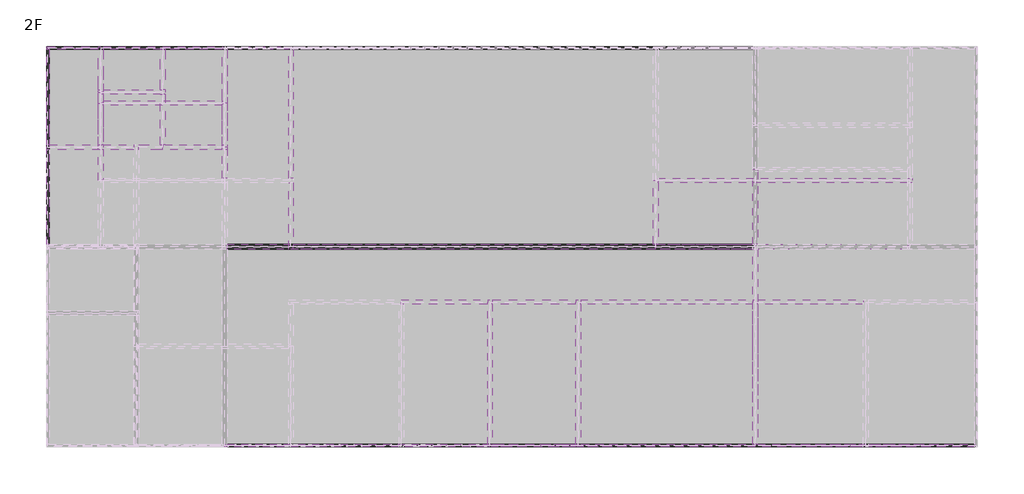
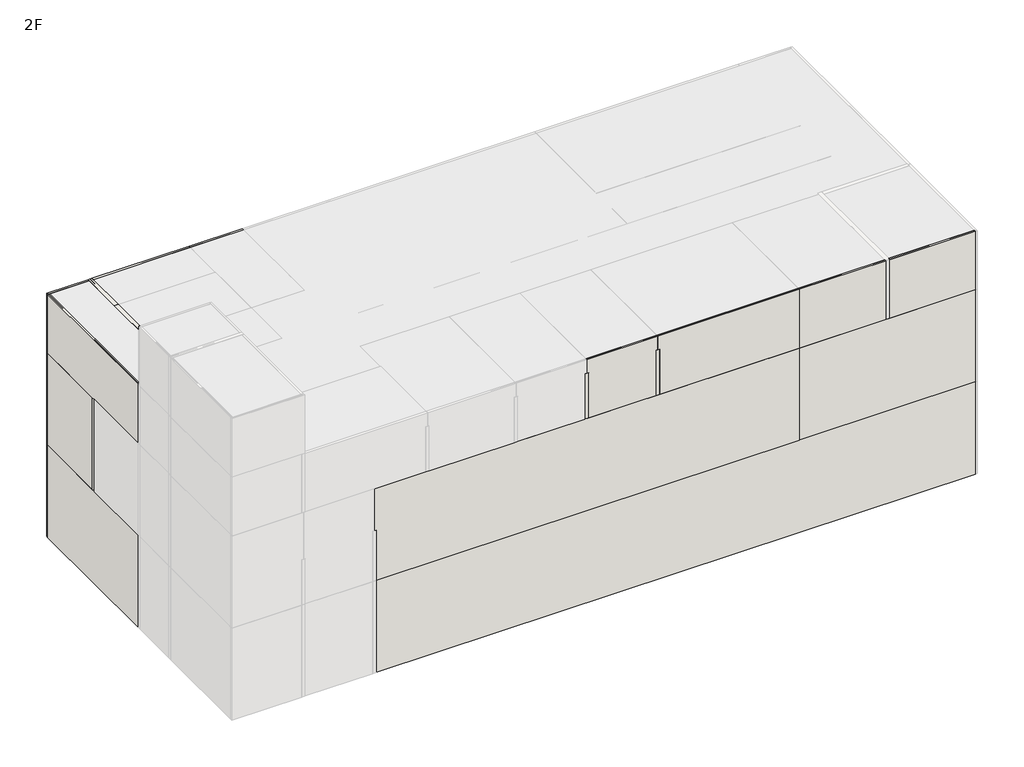
# One storey, part 2 of 3: 49 walls.
"""IFC4 building model written with IfcOpenShell, lengths in millimetres."""

from ifc_helpers import new_model, si_unit, frame, origin, place, context, project, spatial, polyline, outline, extrude, faceted_brep, element, save

model = new_model("IFC4")

# Units and contexts
model_context = context("Model", 3, world=origin())
ifc_project = project(units=[si_unit("LENGTHUNIT", "METRE", prefix="MILLI")], contexts=[model_context])

# Site, building, storey
site = spatial("IfcSite", under=ifc_project)
building = spatial("IfcBuilding", under=site)
storey = spatial("IfcBuildingStorey", under=building, Name="2F", Elevation=3500.0)

# Walls
placement = place(None, origin())
element("IfcWall", 1, ObjectType="WA211_Exterior-Cement Brick-90mm", at=placement, inside=storey, context=model_context, shape_type="Brep", body=[
    faceted_brep([(45402.6521483, 181866.8614395, 3500.0), (45516.6521483, 181866.8614395, 3500.0), (77352.6521483, 181866.8614395, 3500.0), (77352.6521483, 181866.8614395, 9000.0), (45516.6521483, 181866.8614395, 9000.0), (45402.6521483, 181866.8614395, 9000.0), (45402.6521483, 181980.8614395, 3500.0), (45402.6521483, 181980.8614395, 9000.0), (77352.6521483, 181980.8614395, 9000.0), (77352.6521483, 181980.8614395, 3500.0)], [[[0, 1, 2, 3, 4, 5]], [[6, 7, 8, 9]], [[2, 1, 0, 6, 9]], [[5, 4, 3, 8, 7]], [[0, 5, 7, 6]], [[3, 2, 9, 8]]]),
])
element("IfcWall", 2, ObjectType="WA211_Exterior-Cement Brick-90mm", at=placement, inside=storey, context=model_context, shape_type="SweptSolid", body=[
    extrude(outline(polyline([(45516.6521483, 181866.8614395), (45516.6521483, 173030.8614395), (45402.6521483, 173030.8614395), (45402.6521483, 181866.8614395), (45516.6521483, 181866.8614395)])), frame((0.0, 0.0, 3500.0), z_axis=(0.0, 0.0, 1.0), x_axis=(1.0, 0.0, 0.0)), (0.0, 0.0, 1.0), 5500.0),
])
element("IfcWall", 3, ObjectType="WA211_Exterior-Cement Brick-90mm", at=placement, inside=storey, context=model_context, shape_type="SweptSolid", body=[
    extrude(outline(polyline([(53566.6521483, 163980.8614395), (87402.6521483, 163980.8614395), (87402.6521483, 163866.8614395), (53566.6521483, 163866.8614395), (53566.6521483, 163980.8614395)])), frame((0.0, 0.0, 3500.0), z_axis=(0.0, 0.0, 1.0), x_axis=(1.0, 0.0, 0.0)), (0.0, 0.0, 1.0), 5500.0),
])
element("IfcWall", 4, ObjectType="WA211_Exterior-Cement Brick-90mm", at=placement, inside=storey, context=model_context, shape_type="Brep", body=[
    faceted_brep([(77459.6521483, 163980.8614395, 9000.0), (77352.6521483, 163980.8614395, 9000.0), (53566.6521483, 163980.8614395, 9000.0), (53566.6521483, 163980.8614395, 12000.0), (53459.6521483, 163980.8614395, 12000.0), (53459.6521483, 163980.8614395, 14500.0), (77352.6521483, 163980.8614395, 14500.0), (77459.6521483, 163980.8614395, 14500.0), (77459.6521483, 163866.8614395, 9000.0), (77459.6521483, 163866.8614395, 14500.0), (53459.6521483, 163866.8614395, 14500.0), (53459.6521483, 163866.8614395, 12000.0), (53566.6521483, 163866.8614395, 12000.0), (53566.6521483, 163866.8614395, 9000.0)], [[[0, 1, 2, 3, 4, 5, 6, 7]], [[8, 9, 10, 11, 12, 13]], [[2, 1, 0, 8, 13]], [[7, 6, 5, 10, 9]], [[0, 7, 9, 8]], [[5, 4, 11, 10]], [[11, 4, 3, 12]], [[3, 2, 13, 12]]]),
])
element("IfcWall", 5, ObjectType="WA211_Exterior-Cement Brick-90mm", at=placement, inside=storey, context=model_context, shape_type="Brep", body=[
    faceted_brep([(87402.6521483, 163980.8614395, 9000.0), (77566.6521483, 163980.8614395, 9000.0), (77459.6521483, 163980.8614395, 9000.0), (77459.6521483, 163980.8614395, 14500.0), (77566.6521483, 163980.8614395, 14500.0), (87402.6521483, 163980.8614395, 14500.0), (87402.6521483, 163866.8614395, 9000.0), (87402.6521483, 163866.8614395, 14500.0), (77459.6521483, 163866.8614395, 14500.0), (77459.6521483, 163866.8614395, 9000.0)], [[[0, 1, 2, 3, 4, 5]], [[6, 7, 8, 9]], [[2, 1, 0, 6, 9]], [[3, 2, 9, 8]], [[5, 4, 3, 8, 7]], [[0, 5, 7, 6]]]),
])
element("IfcWall", 6, ObjectType="WA211_Exterior-Cement Brick-90mm", at=placement, inside=storey, context=model_context, shape_type="SweptSolid", body=[
    extrude(outline(polyline([(45516.6521483, 181866.8614395), (45516.6521483, 177530.8614395), (45402.6521483, 177530.8614395), (45402.6521483, 181866.8614395), (45516.6521483, 181866.8614395)])), frame((0.0, 0.0, 9000.0), z_axis=(0.0, 0.0, 1.0), x_axis=(1.0, 0.0, 0.0)), (0.0, 0.0, 1.0), 5500.0),
])
element("IfcWall", 7, ObjectType="WA211_Exterior-Cement Brick-90mm", at=placement, inside=storey, context=model_context, shape_type="Brep", body=[
    faceted_brep([(45402.6521483, 181866.8614395, 9000.0), (45516.6521483, 181866.8614395, 9000.0), (47752.6521483, 181866.8614395, 9000.0), (47752.6521483, 181866.8614395, 14500.0), (45516.6521483, 181866.8614395, 14500.0), (45402.6521483, 181866.8614395, 14500.0), (45402.6521483, 181980.8614395, 9000.0), (45402.6521483, 181980.8614395, 14500.0), (47752.6521483, 181980.8614395, 14500.0), (47752.6521483, 181980.8614395, 9000.0)], [[[0, 1, 2, 3, 4, 5]], [[6, 7, 8, 9]], [[2, 1, 0, 6, 9]], [[5, 4, 3, 8, 7]], [[0, 5, 7, 6]], [[3, 2, 9, 8]]]),
])
element("IfcWall", 8, ObjectType="WA211_Exterior-Cement Brick-90mm", at=placement, inside=storey, context=model_context, shape_type="Brep", body=[
    faceted_brep([(50659.6521483, 181866.8614395, 14500.0), (50659.6521483, 181866.8614395, 9000.0), (50766.6521483, 181866.8614395, 9000.0), (53352.6521483, 181866.8614395, 9000.0), (53352.6521483, 181866.8614395, 12400.0), (53459.6521483, 181866.8614395, 12400.0), (53459.6521483, 181866.8614395, 14500.0), (50659.6521483, 181980.8614395, 9000.0), (50659.6521483, 181980.8614395, 14500.0), (53459.6521483, 181980.8614395, 14500.0), (53459.6521483, 181980.8614395, 12400.0), (53352.6521483, 181980.8614395, 12400.0), (53352.6521483, 181980.8614395, 9000.0)], [[[0, 1, 2, 3, 4, 5, 6]], [[7, 8, 9, 10, 11, 12]], [[3, 2, 1, 7, 12]], [[0, 6, 9, 8]], [[6, 5, 10, 9]], [[10, 5, 4, 11]], [[4, 3, 12, 11]], [[0, 8, 7, 1]]]),
])
element("IfcWall", 9, ObjectType="WA211_Exterior-Cement Brick-90mm", at=placement, inside=storey, context=model_context, shape_type="Brep", body=[
    faceted_brep([(47966.6521483, 181866.8614395, 9000.0), (50552.6521483, 181866.8614395, 9000.0), (50659.6521483, 181866.8614395, 9000.0), (50659.6521483, 181866.8614395, 14500.0), (47966.6521483, 181866.8614395, 14500.0), (47966.6521483, 181980.8614395, 9000.0), (47966.6521483, 181980.8614395, 14500.0), (50659.6521483, 181980.8614395, 14500.0), (50659.6521483, 181980.8614395, 9000.0)], [[[0, 1, 2, 3, 4]], [[5, 6, 7, 8]], [[2, 1, 0, 5, 8]], [[4, 3, 7, 6]], [[0, 4, 6, 5]], [[2, 8, 7, 3]]]),
])
element("IfcWall", 10, ObjectType="WA211_Exterior-Cement Brick-90mm", at=placement, inside=storey, context=model_context, shape_type="SweptSolid", body=[
    extrude(outline(polyline([(14500.0, 69352.6521483), (17200.0, 69352.6521483), (17200.0, 69459.6521483), (18000.0, 69459.6521483), (18000.0, 65459.6521483), (17200.0, 65459.6521483), (17200.0, 65566.6521483), (14500.0, 65566.6521483), (14500.0, 69352.6521483)])), frame((0.0, 163866.8614395, 0.0), z_axis=(0.0, 1.0, 0.0), x_axis=(0.0, 0.0, 1.0)), (0.0, 0.0, 1.0), 114.0),
])
element("IfcWall", 11, ObjectType="WA211_Exterior-Cement Brick-90mm", at=placement, inside=storey, context=model_context, shape_type="Brep", body=[
    faceted_brep([(77459.6521483, 163980.8614395, 18000.0), (77459.6521483, 163980.8614395, 14500.0), (77352.6521483, 163980.8614395, 14500.0), (69566.6521483, 163980.8614395, 14500.0), (69566.6521483, 163980.8614395, 17200.0), (69459.6521483, 163980.8614395, 17200.0), (69459.6521483, 163980.8614395, 18000.0), (77459.6521483, 163866.8614395, 14500.0), (77459.6521483, 163866.8614395, 18000.0), (69459.6521483, 163866.8614395, 18000.0), (69459.6521483, 163866.8614395, 17200.0), (69566.6521483, 163866.8614395, 17200.0), (69566.6521483, 163866.8614395, 14500.0)], [[[0, 1, 2, 3, 4, 5, 6]], [[7, 8, 9, 10, 11, 12]], [[3, 2, 1, 7, 12]], [[0, 6, 9, 8]], [[6, 5, 10, 9]], [[10, 5, 4, 11]], [[4, 3, 12, 11]], [[0, 8, 7, 1]]]),
])
element("IfcWall", 12, ObjectType="WA211_Exterior-Cement Brick-90mm", at=placement, inside=storey, context=model_context, shape_type="Brep", body=[
    faceted_brep([(82352.6521483, 163980.8614395, 14500.0), (77566.6521483, 163980.8614395, 14500.0), (77459.6521483, 163980.8614395, 14500.0), (77459.6521483, 163980.8614395, 18000.0), (82352.6521483, 163980.8614395, 18000.0), (82352.6521483, 163866.8614395, 14500.0), (82352.6521483, 163866.8614395, 18000.0), (77459.6521483, 163866.8614395, 18000.0), (77459.6521483, 163866.8614395, 14500.0)], [[[0, 1, 2, 3, 4]], [[5, 6, 7, 8]], [[2, 1, 0, 5, 8]], [[4, 3, 7, 6]], [[2, 8, 7, 3]], [[0, 4, 6, 5]]]),
])
element("IfcWall", 13, ObjectType="WA211_Exterior-Cement Brick-90mm", at=placement, inside=storey, context=model_context, shape_type="SweptSolid", body=[
    extrude(outline(polyline([(82566.6521483, 163980.8614395), (87402.6521483, 163980.8614395), (87402.6521483, 163866.8614395), (82566.6521483, 163866.8614395), (82566.6521483, 163980.8614395)])), frame((0.0, 0.0, 14500.0), z_axis=(0.0, 0.0, 1.0), x_axis=(1.0, 0.0, 0.0)), (0.0, 0.0, 1.0), 3500.0),
])
element("IfcWall", 14, ObjectType="WA211_Exterior-Cement Brick-90mm", at=placement, inside=storey, context=model_context, shape_type="SweptSolid", body=[
    extrude(outline(polyline([(14500.0, 47966.6521483), (14500.0, 53352.6521483), (17200.0, 53352.6521483), (17200.0, 53459.6521483), (18000.0, 53459.6521483), (18000.0, 47966.6521483), (14500.0, 47966.6521483)])), frame((0.0, 181866.8614395, 0.0), z_axis=(0.0, 1.0, 0.0), x_axis=(0.0, 0.0, 1.0)), (0.0, 0.0, 1.0), 114.0),
])
element("IfcWall", 15, ObjectType="WA211_Exterior-Cement Brick-90mm", at=placement, inside=storey, context=model_context, shape_type="SweptSolid", body=[
    extrude(outline(polyline([(14500.0, 53566.6521483), (14500.0, 56352.6521483), (17200.0, 56352.6521483), (17200.0, 56459.6521483), (18000.0, 56459.6521483), (18000.0, 53459.6521483), (17200.0, 53459.6521483), (17200.0, 53566.6521483), (14500.0, 53566.6521483)])), frame((0.0, 181866.8614395, 0.0), z_axis=(0.0, 1.0, 0.0), x_axis=(0.0, 0.0, 1.0)), (0.0, 0.0, 1.0), 114.0),
])
element("IfcWall", 16, ObjectType="WA211_Exterior-Cement Brick-90mm", at=placement, inside=storey, context=model_context, shape_type="Brep", body=[
    faceted_brep([(45402.6521483, 181866.8614395, 14500.0), (45516.6521483, 181866.8614395, 14500.0), (47752.6521483, 181866.8614395, 14500.0), (47752.6521483, 181866.8614395, 18000.0), (45516.6521483, 181866.8614395, 18000.0), (45402.6521483, 181866.8614395, 18000.0), (45402.6521483, 181980.8614395, 14500.0), (45402.6521483, 181980.8614395, 18000.0), (47752.6521483, 181980.8614395, 18000.0), (47752.6521483, 181980.8614395, 14500.0)], [[[0, 1, 2, 3, 4, 5]], [[6, 7, 8, 9]], [[2, 1, 0, 6, 9]], [[5, 4, 3, 8, 7]], [[3, 2, 9, 8]], [[0, 5, 7, 6]]]),
])
element("IfcWall", 17, ObjectType="WA211_Exterior-Cement Brick-90mm", at=placement, inside=storey, context=model_context, shape_type="SweptSolid", body=[
    extrude(outline(polyline([(45516.6521483, 181866.8614395), (45516.6521483, 173030.8614395), (45402.6521483, 173030.8614395), (45402.6521483, 181866.8614395), (45516.6521483, 181866.8614395)])), frame((0.0, 0.0, 14500.0), z_axis=(0.0, 0.0, 1.0), x_axis=(1.0, 0.0, 0.0)), (0.0, 0.0, 1.0), 3500.0),
])
element("IfcWall", 18, ObjectType="WA221_Interior-Cement Block-190mm", at=placement, inside=storey, context=model_context, shape_type="SweptSolid", body=[
    extrude(outline(polyline([(53566.6521483, 173030.8614395), (77352.6521483, 173030.8614395), (77352.6521483, 172816.8614395), (53566.6521483, 172816.8614395), (53566.6521483, 173030.8614395)])), frame((0.0, 0.0, 3500.0), z_axis=(0.0, 0.0, 1.0), x_axis=(1.0, 0.0, 0.0)), (0.0, 0.0, 1.0), 5500.0),
])
element("IfcWall", 19, ObjectType="WA221_Interior-Cement Block-190mm", at=placement, inside=storey, context=model_context, shape_type="Brep", body=[
    faceted_brep([(77459.6521483, 173030.8614395, 9000.0), (77352.6521483, 173030.8614395, 9000.0), (53566.6521483, 173030.8614395, 9000.0), (53566.6521483, 173030.8614395, 12400.0), (77352.6521483, 173030.8614395, 12400.0), (77459.6521483, 173030.8614395, 12400.0), (77459.6521483, 172816.8614395, 9000.0), (77459.6521483, 172816.8614395, 12400.0), (77352.6521483, 172816.8614395, 12400.0), (53566.6521483, 172816.8614395, 12400.0), (53566.6521483, 172816.8614395, 12000.0), (53566.6521483, 172816.8614395, 9000.0), (77352.6521483, 172816.8614395, 9000.0), (53566.6521483, 172923.8614395, 9000.0)], [[[0, 1, 2, 3, 4, 5]], [[6, 7, 8, 9, 10, 11, 12]], [[2, 1, 0, 6, 12, 11, 13]], [[5, 4, 3, 9, 8, 7]], [[0, 5, 7, 6]], [[2, 13, 11, 10, 9, 3]]]),
])
element("IfcWall", 20, ObjectType="WA221_Interior-Cement Block-190mm", at=placement, inside=storey, context=model_context, shape_type="Brep", body=[
    faceted_brep([(77352.6521483, 176316.8614395, 9000.0), (77352.6521483, 173030.8614395, 9000.0), (77352.6521483, 173030.8614395, 12400.0), (77352.6521483, 176423.8614395, 12400.0), (77352.6521483, 176423.8614395, 11700.0), (77352.6521483, 176316.8614395, 11700.0), (77566.6521483, 176316.8614395, 9000.0), (77566.6521483, 176316.8614395, 11700.0), (77566.6521483, 176423.8614395, 11700.0), (77566.6521483, 176423.8614395, 12400.0), (77566.6521483, 173030.8614395, 12400.0), (77566.6521483, 173030.8614395, 9000.0), (77459.6521483, 173030.8614395, 9000.0), (77459.6521483, 173030.8614395, 12400.0)], [[[0, 1, 2, 3, 4, 5]], [[6, 7, 8, 9, 10, 11]], [[1, 0, 6, 11, 12]], [[3, 2, 13, 10, 9]], [[2, 1, 12, 11, 10, 13]], [[4, 3, 9, 8]], [[4, 8, 7, 5]], [[0, 5, 7, 6]]]),
])
element("IfcWall", 21, ObjectType="WA221_Interior-Cement Block-190mm", at=placement, inside=storey, context=model_context, shape_type="Brep", body=[
    faceted_brep([(53566.6521483, 177530.8614395, 9000.0), (53566.6521483, 181866.8614395, 9000.0), (53566.6521483, 181980.8614395, 9000.0), (53566.6521483, 181980.8614395, 12400.0), (53566.6521483, 181866.8614395, 12400.0), (53566.6521483, 177423.8614395, 12400.0), (53566.6521483, 177423.8614395, 11700.0), (53566.6521483, 177530.8614395, 11700.0), (53352.6521483, 177530.8614395, 9000.0), (53352.6521483, 177530.8614395, 11700.0), (53352.6521483, 177423.8614395, 11700.0), (53352.6521483, 177423.8614395, 12400.0), (53352.6521483, 181866.8614395, 12400.0), (53352.6521483, 181980.8614395, 12400.0), (53352.6521483, 181980.8614395, 9000.0), (53352.6521483, 181866.8614395, 9000.0), (53459.6521483, 181980.8614395, 12400.0)], [[[0, 1, 2, 3, 4, 5, 6, 7]], [[8, 9, 10, 11, 12, 13, 14, 15]], [[2, 1, 0, 8, 15, 14]], [[5, 4, 3, 16, 13, 12, 11]], [[3, 2, 14, 13, 16]], [[6, 5, 11, 10]], [[6, 10, 9, 7]], [[0, 7, 9, 8]]]),
])
element("IfcWall", 22, ObjectType="WA221_Interior-Cement Block-190mm", at=placement, inside=storey, context=model_context, shape_type="Brep", body=[
    faceted_brep([(77566.6521483, 163980.8614395, 9000.0), (77566.6521483, 172816.8614395, 9000.0), (77566.6521483, 172816.8614395, 14500.0), (77566.6521483, 163980.8614395, 14500.0), (77352.6521483, 163980.8614395, 9000.0), (77352.6521483, 163980.8614395, 14500.0), (77352.6521483, 172816.8614395, 14500.0), (77352.6521483, 172816.8614395, 12400.0), (77352.6521483, 172816.8614395, 9000.0), (77459.6521483, 163980.8614395, 9000.0), (77459.6521483, 172816.8614395, 9000.0), (77459.6521483, 163980.8614395, 14500.0)], [[[0, 1, 2, 3]], [[4, 5, 6, 7, 8]], [[1, 0, 9, 4, 8, 10]], [[3, 2, 6, 5, 11]], [[1, 10, 8, 7, 6, 2]], [[0, 3, 11, 5, 4, 9]]]),
])
element("IfcWall", 23, ObjectType="WA221_Interior-Cement Block-190mm", at=placement, inside=storey, context=model_context, shape_type="Brep", body=[
    faceted_brep([(47859.6521483, 177530.8614395, 9000.0), (47752.6521483, 177530.8614395, 9000.0), (45516.6521483, 177530.8614395, 9000.0), (45402.6521483, 177530.8614395, 9000.0), (45402.6521483, 177530.8614395, 14500.0), (45516.6521483, 177530.8614395, 14500.0), (47752.6521483, 177530.8614395, 14500.0), (47966.6521483, 177530.8614395, 14500.0), (47966.6521483, 177530.8614395, 11700.0), (47859.6521483, 177530.8614395, 11700.0), (47859.6521483, 177316.8614395, 9000.0), (47859.6521483, 177316.8614395, 11700.0), (47966.6521483, 177316.8614395, 11700.0), (47966.6521483, 177316.8614395, 14500.0), (45516.6521483, 177316.8614395, 14500.0), (45402.6521483, 177316.8614395, 14500.0), (45402.6521483, 177316.8614395, 9000.0), (45516.6521483, 177316.8614395, 9000.0)], [[[0, 1, 2, 3, 4, 5, 6, 7, 8, 9]], [[10, 11, 12, 13, 14, 15, 16, 17]], [[3, 2, 1, 0, 10, 17, 16]], [[7, 6, 5, 4, 15, 14, 13]], [[0, 9, 11, 10]], [[8, 12, 11, 9]], [[8, 7, 13, 12]], [[4, 3, 16, 15]]]),
])
element("IfcWall", 24, ObjectType="WA221_Interior-Cement Block-190mm", at=placement, inside=storey, context=model_context, shape_type="Brep", body=[
    faceted_brep([(47752.6521483, 181980.8614395, 9000.0), (47752.6521483, 181866.8614395, 9000.0), (47752.6521483, 180030.8614395, 9000.0), (47752.6521483, 180030.8614395, 11700.0), (47752.6521483, 179923.8614395, 11700.0), (47752.6521483, 179923.8614395, 14500.0), (47752.6521483, 181866.8614395, 14500.0), (47752.6521483, 181980.8614395, 14500.0), (47966.6521483, 181980.8614395, 9000.0), (47966.6521483, 181980.8614395, 14500.0), (47966.6521483, 181866.8614395, 14500.0), (47966.6521483, 179923.8614395, 14500.0), (47966.6521483, 179923.8614395, 11700.0), (47966.6521483, 180030.8614395, 11700.0), (47966.6521483, 180030.8614395, 9000.0), (47966.6521483, 181866.8614395, 9000.0)], [[[0, 1, 2, 3, 4, 5, 6, 7]], [[8, 9, 10, 11, 12, 13, 14, 15]], [[2, 1, 0, 8, 15, 14]], [[7, 6, 5, 11, 10, 9]], [[0, 7, 9, 8]], [[5, 4, 12, 11]], [[12, 4, 3, 13]], [[3, 2, 14, 13]]]),
])
element("IfcWall", 25, ObjectType="WA221_Interior-Cement Block-190mm", at=placement, inside=storey, context=model_context, shape_type="Brep", body=[
    faceted_brep([(47752.6521483, 179816.8614395, 9000.0), (47752.6521483, 177530.8614395, 9000.0), (47752.6521483, 177530.8614395, 14500.0), (47752.6521483, 179923.8614395, 14500.0), (47752.6521483, 179923.8614395, 11700.0), (47752.6521483, 179816.8614395, 11700.0), (47966.6521483, 179816.8614395, 9000.0), (47966.6521483, 179816.8614395, 11700.0), (47966.6521483, 179923.8614395, 11700.0), (47966.6521483, 179923.8614395, 14500.0), (47966.6521483, 177530.8614395, 14500.0), (47966.6521483, 177530.8614395, 11700.0), (47966.6521483, 177530.8614395, 9000.0), (47859.6521483, 177530.8614395, 9000.0)], [[[0, 1, 2, 3, 4, 5]], [[6, 7, 8, 9, 10, 11, 12]], [[1, 0, 6, 12, 13]], [[3, 2, 10, 9]], [[1, 13, 12, 11, 10, 2]], [[4, 3, 9, 8]], [[4, 8, 7, 5]], [[0, 5, 7, 6]]]),
])
element("IfcWall", 26, ObjectType="WA221_Interior-Cement Block-190mm", at=placement, inside=storey, context=model_context, shape_type="Brep", body=[
    faceted_brep([(49352.6521483, 177530.8614395, 9000.0), (47966.6521483, 177530.8614395, 9000.0), (47859.6521483, 177530.8614395, 9000.0), (47859.6521483, 177530.8614395, 11700.0), (47966.6521483, 177530.8614395, 11700.0), (49352.6521483, 177530.8614395, 11700.0), (49352.6521483, 177316.8614395, 9000.0), (49352.6521483, 177316.8614395, 11700.0), (47966.6521483, 177316.8614395, 11700.0), (47859.6521483, 177316.8614395, 11700.0), (47859.6521483, 177316.8614395, 9000.0)], [[[0, 1, 2, 3, 4, 5]], [[6, 7, 8, 9, 10]], [[2, 1, 0, 6, 10]], [[3, 2, 10, 9]], [[5, 4, 3, 9, 8, 7]], [[0, 5, 7, 6]]]),
])
element("IfcWall", 27, ObjectType="WA221_Interior-Cement Block-190mm", at=placement, inside=storey, context=model_context, shape_type="Brep", body=[
    faceted_brep([(50552.6521483, 181866.8614395, 9000.0), (50552.6521483, 180030.8614395, 9000.0), (50552.6521483, 180030.8614395, 11700.0), (50552.6521483, 181866.8614395, 11700.0), (50766.6521483, 181866.8614395, 9000.0), (50766.6521483, 181866.8614395, 11700.0), (50766.6521483, 180030.8614395, 11700.0), (50766.6521483, 180030.8614395, 9000.0), (50659.6521483, 181866.8614395, 9000.0)], [[[0, 1, 2, 3]], [[4, 5, 6, 7]], [[1, 0, 8, 4, 7]], [[3, 2, 6, 5]], [[0, 3, 5, 4, 8]], [[2, 1, 7, 6]]]),
])
element("IfcWall", 28, ObjectType="WA221_Interior-Cement Block-190mm", at=placement, inside=storey, context=model_context, shape_type="Brep", body=[
    faceted_brep([(50766.6521483, 177530.8614395, 9000.0), (50766.6521483, 179816.8614395, 9000.0), (50766.6521483, 179816.8614395, 11700.0), (50766.6521483, 177530.8614395, 11700.0), (50552.6521483, 177530.8614395, 9000.0), (50552.6521483, 177530.8614395, 11700.0), (50552.6521483, 179816.8614395, 11700.0), (50552.6521483, 179816.8614395, 9000.0), (50659.6521483, 177530.8614395, 9000.0), (50659.6521483, 177530.8614395, 11700.0)], [[[0, 1, 2, 3]], [[4, 5, 6, 7]], [[1, 0, 8, 4, 7]], [[3, 2, 6, 5, 9]], [[0, 3, 9, 5, 4, 8]], [[2, 1, 7, 6]]]),
])
element("IfcWall", 29, ObjectType="WA221_Interior-Cement Block-190mm", at=placement, inside=storey, context=model_context, shape_type="Brep", body=[
    faceted_brep([(50659.6521483, 177316.8614395, 9000.0), (53352.6521483, 177316.8614395, 9000.0), (53566.6521483, 177316.8614395, 9000.0), (53566.6521483, 177316.8614395, 11700.0), (53352.6521483, 177316.8614395, 11700.0), (50659.6521483, 177316.8614395, 11700.0), (50659.6521483, 177530.8614395, 9000.0), (50659.6521483, 177530.8614395, 11700.0), (50766.6521483, 177530.8614395, 11700.0), (53352.6521483, 177530.8614395, 11700.0), (53566.6521483, 177530.8614395, 11700.0), (53566.6521483, 177530.8614395, 9000.0), (53352.6521483, 177530.8614395, 9000.0), (50766.6521483, 177530.8614395, 9000.0), (53566.6521483, 177423.8614395, 11700.0)], [[[0, 1, 2, 3, 4, 5]], [[6, 7, 8, 9, 10, 11, 12, 13]], [[2, 1, 0, 6, 13, 12, 11]], [[5, 4, 3, 14, 10, 9, 8, 7]], [[0, 5, 7, 6]], [[3, 2, 11, 10, 14]]]),
])
element("IfcWall", 30, ObjectType="WA221_Interior-Cement Block-190mm", at=placement, inside=storey, context=model_context, shape_type="Brep", body=[
    faceted_brep([(50766.6521483, 180030.8614395, 9000.0), (50552.6521483, 180030.8614395, 9000.0), (47966.6521483, 180030.8614395, 9000.0), (47752.6521483, 180030.8614395, 9000.0), (47752.6521483, 180030.8614395, 11700.0), (47966.6521483, 180030.8614395, 11700.0), (50552.6521483, 180030.8614395, 11700.0), (50766.6521483, 180030.8614395, 11700.0), (50766.6521483, 179816.8614395, 9000.0), (50766.6521483, 179816.8614395, 11700.0), (50552.6521483, 179816.8614395, 11700.0), (47966.6521483, 179816.8614395, 11700.0), (47752.6521483, 179816.8614395, 11700.0), (47752.6521483, 179816.8614395, 9000.0), (47966.6521483, 179816.8614395, 9000.0), (50552.6521483, 179816.8614395, 9000.0), (47752.6521483, 179923.8614395, 11700.0)], [[[0, 1, 2, 3, 4, 5, 6, 7]], [[8, 9, 10, 11, 12, 13, 14, 15]], [[3, 2, 1, 0, 8, 15, 14, 13]], [[7, 6, 5, 4, 16, 12, 11, 10, 9]], [[0, 7, 9, 8]], [[4, 3, 13, 12, 16]]]),
])
element("IfcWall", 31, ObjectType="WA221_Interior-Cement Block-190mm", at=placement, inside=storey, context=model_context, shape_type="Brep", body=[
    faceted_brep([(50659.6521483, 177530.8614395, 9000.0), (50552.6521483, 177530.8614395, 9000.0), (49566.6521483, 177530.8614395, 9000.0), (49566.6521483, 177530.8614395, 11700.0), (50552.6521483, 177530.8614395, 11700.0), (50659.6521483, 177530.8614395, 11700.0), (50659.6521483, 177316.8614395, 9000.0), (50659.6521483, 177316.8614395, 11700.0), (49566.6521483, 177316.8614395, 11700.0), (49566.6521483, 177316.8614395, 9000.0)], [[[0, 1, 2, 3, 4, 5]], [[6, 7, 8, 9]], [[2, 1, 0, 6, 9]], [[5, 4, 3, 8, 7]], [[0, 5, 7, 6]], [[3, 2, 9, 8]]]),
])
element("IfcWall", 32, ObjectType="WA221_Interior-Cement Block-190mm", at=placement, inside=storey, context=model_context, shape_type="Brep", body=[
    faceted_brep([(65352.6521483, 170530.8614395, 14500.0), (65352.6521483, 170316.8614395, 14500.0), (65352.6521483, 163980.8614395, 14500.0), (65352.6521483, 163866.8614395, 14500.0), (65352.6521483, 163866.8614395, 17200.0), (65352.6521483, 163980.8614395, 17200.0), (65352.6521483, 170316.8614395, 17200.0), (65352.6521483, 170530.8614395, 17200.0), (65566.6521483, 170530.8614395, 14500.0), (65566.6521483, 170530.8614395, 17200.0), (65566.6521483, 170316.8614395, 17200.0), (65566.6521483, 163980.8614395, 17200.0), (65566.6521483, 163866.8614395, 17200.0), (65566.6521483, 163866.8614395, 14500.0), (65566.6521483, 163980.8614395, 14500.0), (65566.6521483, 170316.8614395, 14500.0), (65459.6521483, 163866.8614395, 17200.0)], [[[0, 1, 2, 3, 4, 5, 6, 7]], [[8, 9, 10, 11, 12, 13, 14, 15]], [[3, 2, 1, 0, 8, 15, 14, 13]], [[7, 6, 5, 4, 16, 12, 11, 10, 9]], [[4, 3, 13, 12, 16]], [[0, 7, 9, 8]]]),
])
element("IfcWall", 33, ObjectType="WA221_Interior-Cement Block-190mm", at=placement, inside=storey, context=model_context, shape_type="Brep", body=[
    faceted_brep([(61459.6521483, 170316.8614395, 14500.0), (61566.6521483, 170316.8614395, 14500.0), (65352.6521483, 170316.8614395, 14500.0), (65352.6521483, 170316.8614395, 17200.0), (61566.6521483, 170316.8614395, 17200.0), (61459.6521483, 170316.8614395, 17200.0), (61459.6521483, 170530.8614395, 14500.0), (61459.6521483, 170530.8614395, 17200.0), (65352.6521483, 170530.8614395, 17200.0), (65352.6521483, 170530.8614395, 14500.0)], [[[0, 1, 2, 3, 4, 5]], [[6, 7, 8, 9]], [[2, 1, 0, 6, 9]], [[5, 4, 3, 8, 7]], [[0, 5, 7, 6]], [[3, 2, 9, 8]]]),
])
element("IfcWall", 34, ObjectType="WA221_Interior-Cement Block-190mm", at=placement, inside=storey, context=model_context, shape_type="Brep", body=[
    faceted_brep([(69566.6521483, 163866.8614395, 14500.0), (69566.6521483, 163980.8614395, 14500.0), (69566.6521483, 170316.8614395, 14500.0), (69566.6521483, 170530.8614395, 14500.0), (69566.6521483, 170530.8614395, 17200.0), (69566.6521483, 170316.8614395, 17200.0), (69566.6521483, 163980.8614395, 17200.0), (69566.6521483, 163866.8614395, 17200.0), (69352.6521483, 163866.8614395, 14500.0), (69352.6521483, 163866.8614395, 17200.0), (69352.6521483, 163980.8614395, 17200.0), (69352.6521483, 170316.8614395, 17200.0), (69352.6521483, 170530.8614395, 17200.0), (69352.6521483, 170530.8614395, 14500.0), (69352.6521483, 170316.8614395, 14500.0), (69352.6521483, 163980.8614395, 14500.0), (69459.6521483, 163866.8614395, 17200.0)], [[[0, 1, 2, 3, 4, 5, 6, 7]], [[8, 9, 10, 11, 12, 13, 14, 15]], [[3, 2, 1, 0, 8, 15, 14, 13]], [[7, 6, 5, 4, 12, 11, 10, 9, 16]], [[4, 3, 13, 12]], [[0, 7, 16, 9, 8]]]),
])
element("IfcWall", 35, ObjectType="WA221_Interior-Cement Block-190mm", at=placement, inside=storey, context=model_context, shape_type="SweptSolid", body=[
    extrude(outline(polyline([(65566.6521483, 170530.8614395), (69352.6521483, 170530.8614395), (69352.6521483, 170316.8614395), (65566.6521483, 170316.8614395), (65566.6521483, 170530.8614395)])), frame((0.0, 0.0, 14500.0), z_axis=(0.0, 0.0, 1.0), x_axis=(1.0, 0.0, 0.0)), (0.0, 0.0, 1.0), 2700.0),
])
element("IfcWall", 36, ObjectType="WA221_Interior-Cement Block-190mm", at=placement, inside=storey, context=model_context, shape_type="Brep", body=[
    faceted_brep([(84566.6521483, 176030.8614395, 14500.0), (84352.6521483, 176030.8614395, 14500.0), (73066.6521483, 176030.8614395, 14500.0), (73066.6521483, 176030.8614395, 17200.0), (84352.6521483, 176030.8614395, 17200.0), (84566.6521483, 176030.8614395, 17200.0), (84566.6521483, 175816.8614395, 14500.0), (84566.6521483, 175816.8614395, 17200.0), (84352.6521483, 175816.8614395, 17200.0), (73066.6521483, 175816.8614395, 17200.0), (73066.6521483, 175816.8614395, 14500.0), (84352.6521483, 175816.8614395, 14500.0), (73066.6521483, 175923.8614395, 14500.0), (73066.6521483, 175923.8614395, 17200.0)], [[[0, 1, 2, 3, 4, 5]], [[6, 7, 8, 9, 10, 11]], [[2, 1, 0, 6, 11, 10, 12]], [[5, 4, 3, 13, 9, 8, 7]], [[0, 5, 7, 6]], [[3, 2, 12, 10, 9, 13]]]),
])
element("IfcWall", 37, ObjectType="WA221_Interior-Cement Block-190mm", at=placement, inside=storey, context=model_context, shape_type="Brep", body=[
    faceted_brep([(77352.6521483, 170530.8614395, 14500.0), (77352.6521483, 170316.8614395, 14500.0), (77352.6521483, 163980.8614395, 14500.0), (77352.6521483, 163980.8614395, 17200.0), (77352.6521483, 170316.8614395, 17200.0), (77352.6521483, 170530.8614395, 17200.0), (77566.6521483, 170530.8614395, 14500.0), (77566.6521483, 170530.8614395, 17200.0), (77566.6521483, 170316.8614395, 17200.0), (77566.6521483, 163980.8614395, 17200.0), (77566.6521483, 163980.8614395, 14500.0), (77566.6521483, 170316.8614395, 14500.0), (77459.6521483, 163980.8614395, 14500.0)], [[[0, 1, 2, 3, 4, 5]], [[6, 7, 8, 9, 10, 11]], [[2, 1, 0, 6, 11, 10, 12]], [[5, 4, 3, 9, 8, 7]], [[0, 5, 7, 6]], [[3, 2, 12, 10, 9]]]),
])
element("IfcWall", 38, ObjectType="WA221_Interior-Cement Block-190mm", at=placement, inside=storey, context=model_context, shape_type="SweptSolid", body=[
    extrude(outline(polyline([(77352.6521483, 170316.8614395), (69566.6521483, 170316.8614395), (69566.6521483, 170530.8614395), (77352.6521483, 170530.8614395), (77352.6521483, 170316.8614395)])), frame((0.0, 0.0, 14500.0), z_axis=(0.0, 0.0, 1.0), x_axis=(1.0, 0.0, 0.0)), (0.0, 0.0, 1.0), 2700.0),
])
element("IfcWall", 39, ObjectType="WA221_Interior-Cement Block-190mm", at=placement, inside=storey, context=model_context, shape_type="Brep", body=[
    faceted_brep([(73066.6521483, 173030.8614395, 14500.0), (73066.6521483, 175816.8614395, 14500.0), (73066.6521483, 175923.8614395, 14500.0), (73066.6521483, 175923.8614395, 17200.0), (73066.6521483, 175816.8614395, 17200.0), (73066.6521483, 173030.8614395, 17200.0), (72852.6521483, 173030.8614395, 14500.0), (72852.6521483, 173030.8614395, 17200.0), (72852.6521483, 175923.8614395, 17200.0), (72852.6521483, 175923.8614395, 14500.0), (72959.6521483, 173030.8614395, 14500.0), (72959.6521483, 173030.8614395, 17200.0)], [[[0, 1, 2, 3, 4, 5]], [[6, 7, 8, 9]], [[2, 1, 0, 10, 6, 9]], [[3, 2, 9, 8]], [[5, 4, 3, 8, 7, 11]], [[0, 5, 11, 7, 6, 10]]]),
])
element("IfcWall", 40, ObjectType="WA221_Interior-Cement Block-190mm", at=placement, inside=storey, context=model_context, shape_type="Brep", body=[
    faceted_brep([(56352.6521483, 181980.8614395, 14500.0), (56352.6521483, 181866.8614395, 14500.0), (56352.6521483, 176030.8614395, 14500.0), (56352.6521483, 176030.8614395, 17200.0), (56352.6521483, 181866.8614395, 17200.0), (56352.6521483, 181980.8614395, 17200.0), (56566.6521483, 181980.8614395, 14500.0), (56566.6521483, 181980.8614395, 17200.0), (56566.6521483, 181866.8614395, 17200.0), (56566.6521483, 176030.8614395, 17200.0), (56566.6521483, 176030.8614395, 14500.0), (56566.6521483, 181866.8614395, 14500.0), (56459.6521483, 181980.8614395, 17200.0)], [[[0, 1, 2, 3, 4, 5]], [[6, 7, 8, 9, 10, 11]], [[2, 1, 0, 6, 11, 10]], [[5, 4, 3, 9, 8, 7, 12]], [[0, 5, 12, 7, 6]], [[3, 2, 10, 9]]]),
])
element("IfcWall", 41, ObjectType="WA221_Interior-Cement Block-190mm", at=placement, inside=storey, context=model_context, shape_type="Brep", body=[
    faceted_brep([(56566.6521483, 172816.8614395, 14500.0), (56566.6521483, 173030.8614395, 14500.0), (56566.6521483, 175816.8614395, 14500.0), (56566.6521483, 175816.8614395, 17200.0), (56566.6521483, 173030.8614395, 17200.0), (56566.6521483, 172816.8614395, 17200.0), (56352.6521483, 172816.8614395, 14500.0), (56352.6521483, 172816.8614395, 17200.0), (56352.6521483, 175816.8614395, 17200.0), (56352.6521483, 175816.8614395, 14500.0)], [[[0, 1, 2, 3, 4, 5]], [[6, 7, 8, 9]], [[2, 1, 0, 6, 9]], [[5, 4, 3, 8, 7]], [[0, 5, 7, 6]], [[3, 2, 9, 8]]]),
])
element("IfcWall", 42, ObjectType="WA221_Interior-Cement Block-190mm", at=placement, inside=storey, context=model_context, shape_type="Brep", body=[
    faceted_brep([(72959.6521483, 173030.8614395, 14500.0), (72852.6521483, 173030.8614395, 14500.0), (56566.6521483, 173030.8614395, 14500.0), (56566.6521483, 173030.8614395, 17200.0), (72852.6521483, 173030.8614395, 17200.0), (72959.6521483, 173030.8614395, 17200.0), (72959.6521483, 172816.8614395, 14500.0), (72959.6521483, 172816.8614395, 17200.0), (56566.6521483, 172816.8614395, 17200.0), (56566.6521483, 172816.8614395, 14500.0)], [[[0, 1, 2, 3, 4, 5]], [[6, 7, 8, 9]], [[2, 1, 0, 6, 9]], [[5, 4, 3, 8, 7]], [[0, 5, 7, 6]], [[3, 2, 9, 8]]]),
])
element("IfcWall", 43, ObjectType="WA221_Interior-Cement Block-190mm", at=placement, inside=storey, context=model_context, shape_type="SweptSolid", body=[
    extrude(outline(polyline([(82352.6521483, 170316.8614395), (77566.6521483, 170316.8614395), (77566.6521483, 170530.8614395), (82352.6521483, 170530.8614395), (82352.6521483, 170316.8614395)])), frame((0.0, 0.0, 14500.0), z_axis=(0.0, 0.0, 1.0), x_axis=(1.0, 0.0, 0.0)), (0.0, 0.0, 1.0), 2700.0),
])
element("IfcWall", 44, ObjectType="WA221_Interior-Cement Block-190mm", at=placement, inside=storey, context=model_context, shape_type="Brep", body=[
    faceted_brep([(84352.6521483, 173030.8614395, 14500.0), (73066.6521483, 173030.8614395, 14500.0), (72959.6521483, 173030.8614395, 14500.0), (72959.6521483, 173030.8614395, 17200.0), (73066.6521483, 173030.8614395, 17200.0), (84352.6521483, 173030.8614395, 17200.0), (84352.6521483, 172816.8614395, 14500.0), (84352.6521483, 172816.8614395, 17200.0), (72959.6521483, 172816.8614395, 17200.0), (72959.6521483, 172816.8614395, 14500.0)], [[[0, 1, 2, 3, 4, 5]], [[6, 7, 8, 9]], [[2, 1, 0, 6, 9]], [[3, 2, 9, 8]], [[5, 4, 3, 8, 7]], [[0, 5, 7, 6]]]),
])
element("IfcWall", 45, ObjectType="WA221_Interior-Cement Block-190mm", at=placement, inside=storey, context=model_context, shape_type="Brep", body=[
    faceted_brep([(53352.6521483, 179530.8614395, 14500.0), (47966.6521483, 179530.8614395, 14500.0), (47966.6521483, 179530.8614395, 17200.0), (53352.6521483, 179530.8614395, 17200.0), (53352.6521483, 179316.8614395, 14500.0), (53352.6521483, 179316.8614395, 17200.0), (47966.6521483, 179316.8614395, 17200.0), (47966.6521483, 179316.8614395, 14500.0), (53352.6521483, 179423.8614395, 14500.0), (47966.6521483, 179423.8614395, 14500.0), (53352.6521483, 179423.8614395, 17200.0)], [[[0, 1, 2, 3]], [[4, 5, 6, 7]], [[1, 0, 8, 4, 7, 9]], [[3, 2, 6, 5, 10]], [[0, 3, 10, 5, 4, 8]], [[2, 1, 9, 7, 6]]]),
])
element("IfcWall", 46, ObjectType="WA221_Interior-Cement Block-190mm", at=placement, inside=storey, context=model_context, shape_type="Brep", body=[
    faceted_brep([(53352.6521483, 179423.8614395, 14500.0), (53352.6521483, 179316.8614395, 14500.0), (53352.6521483, 176030.8614395, 14500.0), (53352.6521483, 176030.8614395, 17200.0), (53352.6521483, 179316.8614395, 17200.0), (53352.6521483, 179423.8614395, 17200.0), (53566.6521483, 179423.8614395, 14500.0), (53566.6521483, 179423.8614395, 17200.0), (53566.6521483, 176030.8614395, 17200.0), (53566.6521483, 176030.8614395, 14500.0), (53459.6521483, 176030.8614395, 14500.0), (53459.6521483, 176030.8614395, 17200.0)], [[[0, 1, 2, 3, 4, 5]], [[6, 7, 8, 9]], [[2, 1, 0, 6, 9, 10]], [[5, 4, 3, 11, 8, 7]], [[0, 5, 7, 6]], [[3, 2, 10, 9, 8, 11]]]),
])
element("IfcWall", 47, ObjectType="WA221_Interior-Cement Block-190mm", at=placement, inside=storey, context=model_context, shape_type="Brep", body=[
    faceted_brep([(47752.6521483, 179423.8614395, 18000.0), (47752.6521483, 179423.8614395, 14500.0), (47752.6521483, 175923.8614395, 14500.0), (47752.6521483, 175923.8614395, 18000.0), (47966.6521483, 179423.8614395, 14500.0), (47966.6521483, 179423.8614395, 18000.0), (47966.6521483, 175923.8614395, 18000.0), (47966.6521483, 175923.8614395, 14500.0), (47966.6521483, 176030.8614395, 14500.0), (47966.6521483, 179316.8614395, 14500.0)], [[[0, 1, 2, 3]], [[4, 5, 6, 7, 8, 9]], [[2, 1, 4, 9, 8, 7]], [[0, 3, 6, 5]], [[0, 5, 4, 1]], [[2, 7, 6, 3]]]),
])
element("IfcWall", 48, ObjectType="WA221_Interior-Cement Block-190mm", at=placement, inside=storey, context=model_context, shape_type="Brep", body=[
    faceted_brep([(53352.6521483, 181980.8614395, 14500.0), (53352.6521483, 181866.8614395, 14500.0), (53352.6521483, 179530.8614395, 14500.0), (53352.6521483, 179423.8614395, 14500.0), (53352.6521483, 179423.8614395, 17200.0), (53352.6521483, 179530.8614395, 17200.0), (53352.6521483, 181866.8614395, 17200.0), (53352.6521483, 181980.8614395, 17200.0), (53566.6521483, 181980.8614395, 14500.0), (53566.6521483, 181980.8614395, 17200.0), (53566.6521483, 181866.8614395, 17200.0), (53566.6521483, 179423.8614395, 17200.0), (53566.6521483, 179423.8614395, 14500.0), (53566.6521483, 181866.8614395, 14500.0), (53459.6521483, 181980.8614395, 17200.0)], [[[0, 1, 2, 3, 4, 5, 6, 7]], [[8, 9, 10, 11, 12, 13]], [[3, 2, 1, 0, 8, 13, 12]], [[4, 3, 12, 11]], [[7, 6, 5, 4, 11, 10, 9, 14]], [[0, 7, 14, 9, 8]]]),
])
element("IfcWall", 49, ObjectType="WA221_Interior-Cement Block-190mm", at=placement, inside=storey, context=model_context, shape_type="Brep", body=[
    faceted_brep([(47752.6521483, 181980.8614395, 14500.0), (47752.6521483, 181866.8614395, 14500.0), (47752.6521483, 179423.8614395, 14500.0), (47752.6521483, 179423.8614395, 18000.0), (47752.6521483, 181866.8614395, 18000.0), (47752.6521483, 181980.8614395, 18000.0), (47966.6521483, 181980.8614395, 14500.0), (47966.6521483, 181980.8614395, 18000.0), (47966.6521483, 181866.8614395, 18000.0), (47966.6521483, 179423.8614395, 18000.0), (47966.6521483, 179423.8614395, 14500.0), (47966.6521483, 179530.8614395, 14500.0), (47966.6521483, 181866.8614395, 14500.0)], [[[0, 1, 2, 3, 4, 5]], [[6, 7, 8, 9, 10, 11, 12]], [[2, 1, 0, 6, 12, 11, 10]], [[5, 4, 3, 9, 8, 7]], [[2, 10, 9, 3]], [[0, 5, 7, 6]]]),
])

save(model, "model.ifc")

# Revit data of these elements
# Type "WA211_Exterior-Cement Brick-90mm"
#   Type Comments = ""
#   Layers, outside or top first: 0 mm "A04AL081-00001_Skirt_Acrylic Emulsion Paint" (function 100); 0 mm "A04AL077-00001_Ext Wall Painting_Acrylic Emulsion Paint" (function 100); 12 mm "A04AS164-00001_Plastering_Ext" (function 4); 90 mm "A04AK073-00001_Concrete Brick_0.5B" (function 1); 12 mm "A04AS164-00002_Plastering_Int" (function 5); 0 mm "A04AL078-00002_Int Wall Painting_Water Emulsion Paint" (function 100); 0 mm "A04AL081-00001_Skirt_Acrylic Emulsion Paint" (function 100)
# Type "WA221_Interior-Cement Block-190mm"
#   Type Comments = ""
#   Layers, outside or top first: 0 mm "A04AL081-00001_Skirt_Acrylic Emulsion Paint" (function 100); 0 mm "A04AL078-00002_Int Wall Painting_Water Emulsion Paint" (function 100); 12 mm "A04AS164-00002_Plastering_Int" (function 2); 190 mm "A04AK069-00002_Reinforced Concrete Block_THK 100-200mm" (function 1); 12 mm "A04AS164-00002_Plastering_Int" (function 2); 0 mm "A04AL078-00002_Int Wall Painting_Water Emulsion Paint" (function 100); 0 mm "A04AL081-00001_Skirt_Acrylic Emulsion Paint" (function 100)
# Element 1 (IfcWall, "WA211_Exterior-Cement Brick-90mm")
#   Top Offset = 0 mm
#   Base Offset = 0 mm
#   Unconnected Height = 5500 mm
#   wall height = 5500 mm
#   Phase Created = New Construction
#   Base Constraint = 2F
#   Materials on its faces: "Default Wall", "A04AS164-00001_Plastering_Ext", "A04AS164-00002_Plastering_Int"
# Elements 2, 3 (IfcWall, "WA211_Exterior-Cement Brick-90mm")
#   Top Offset = 0 mm
#   Base Offset = 0 mm
#   Unconnected Height = 5500 mm
#   wall height = 5500 mm
#   Phase Created = New Construction
#   Base Constraint = 2F
#   Materials on its faces: "Default Wall", "A04AS164-00002_Plastering_Int", "A04AS164-00001_Plastering_Ext"
# Elements 4, 5, 6, 8, 9 (IfcWall, "WA211_Exterior-Cement Brick-90mm")
#   Top Offset = 0 mm
#   Base Offset = 0 mm
#   Unconnected Height = 5500 mm
#   wall height = 5500 mm
#   Phase Created = New Construction
#   Base Constraint = 3F
#   Materials on its faces: "Default Wall", "A04AS164-00002_Plastering_Int", "A04AS164-00001_Plastering_Ext"
# Element 7 (IfcWall, "WA211_Exterior-Cement Brick-90mm")
#   Top Offset = 0 mm
#   Base Offset = 0 mm
#   Unconnected Height = 5500 mm
#   wall height = 5500 mm
#   Phase Created = New Construction
#   Base Constraint = 3F
#   Materials on its faces: "Default Wall", "A04AS164-00001_Plastering_Ext", "A04AS164-00002_Plastering_Int"
# Elements 10, 11, 12, 13, 14, 15, 17 (IfcWall, "WA211_Exterior-Cement Brick-90mm")
#   Top Offset = 0 mm
#   Base Offset = 0 mm
#   Unconnected Height = 3500 mm
#   wall height = 3500 mm
#   Phase Created = New Construction
#   Base Constraint = 4F
#   Materials on its faces: "Default Wall", "A04AS164-00002_Plastering_Int", "A04AS164-00001_Plastering_Ext"
# Element 16 (IfcWall, "WA211_Exterior-Cement Brick-90mm")
#   Top Offset = 0 mm
#   Base Offset = 0 mm
#   Unconnected Height = 3500 mm
#   wall height = 3500 mm
#   Phase Created = New Construction
#   Base Constraint = 4F
#   Materials on its faces: "Default Wall", "A04AS164-00001_Plastering_Ext", "A04AS164-00002_Plastering_Int"
# Element 18 (IfcWall, "WA221_Interior-Cement Block-190mm")
#   Top Offset = 0 mm
#   Base Offset = 0 mm
#   Unconnected Height = 5500 mm
#   wall height = 5500 mm
#   Phase Created = New Construction
#   Base Constraint = 2F
#   Materials on its faces: "Default Wall", "A04AS164-00002_Plastering_Int"
# Elements 19, 20 (IfcWall, "WA221_Interior-Cement Block-190mm")
#   Top Offset = 0 mm
#   Base Offset = 0 mm
#   Unconnected Height = 3400 mm
#   wall height = 3400 mm
#   Phase Created = New Construction
#   Base Constraint = 3F
#   Materials on its faces: "Default Wall", "A04AS164-00002_Plastering_Int"
# Element 21 (IfcWall, "WA221_Interior-Cement Block-190mm")
#   Top Offset = 0 mm
#   Base Offset = 0 mm
#   Unconnected Height = 3400 mm
#   wall height = 3400 mm
#   Phase Created = New Construction
#   Base Constraint = 3F
#   Materials on its faces: "Default Wall", "A04AS164-00002_Plastering_Int", "A04AS164-00001_Plastering_Ext"
# Elements 22, 25 (IfcWall, "WA221_Interior-Cement Block-190mm")
#   Top Offset = 0 mm
#   Base Offset = 0 mm
#   Unconnected Height = 5500 mm
#   wall height = 5500 mm
#   Phase Created = New Construction
#   Base Constraint = 3F
#   Materials on its faces: "Default Wall", "A04AS164-00002_Plastering_Int"
# Elements 23, 24 (IfcWall, "WA221_Interior-Cement Block-190mm")
#   Top Offset = 0 mm
#   Base Offset = 0 mm
#   Unconnected Height = 5500 mm
#   wall height = 5500 mm
#   Phase Created = New Construction
#   Base Constraint = 3F
#   Materials on its faces: "Default Wall", "A04AS164-00002_Plastering_Int", "A04AS164-00001_Plastering_Ext"
# Elements 26, 27, 28, 31 (IfcWall, "WA221_Interior-Cement Block-190mm")
#   Top Offset = 0 mm
#   Base Offset = 0 mm
#   Unconnected Height = 2700 mm
#   wall height = 2700 mm
#   Phase Created = New Construction
#   Base Constraint = 3F
#   Materials on its faces: "Default Wall", "A04AS164-00002_Plastering_Int"
# Elements 29, 30 (IfcWall, "WA221_Interior-Cement Block-190mm")
#   Top Offset = 0 mm
#   Base Offset = 0 mm
#   Unconnected Height = 2700 mm
#   wall height = 2700 mm
#   Phase Created = New Construction
#   Base Constraint = 3F
#   Materials on its faces: "A04AS164-00002_Plastering_Int", "Default Wall"
# Elements 32, 34 (IfcWall, "WA221_Interior-Cement Block-190mm")
#   Top Offset = 0 mm
#   Base Offset = 0 mm
#   Unconnected Height = 2700 mm
#   wall height = 2700 mm
#   Phase Created = New Construction
#   Base Constraint = 4F
#   Materials on its faces: "A04AS164-00002_Plastering_Int", "Default Wall", "A04AS164-00001_Plastering_Ext"
# Elements 33, 35, 38, 39, 42, 43, 44, 45, 46 (IfcWall, "WA221_Interior-Cement Block-190mm")
#   Top Offset = 0 mm
#   Base Offset = 0 mm
#   Unconnected Height = 2700 mm
#   wall height = 2700 mm
#   Phase Created = New Construction
#   Base Constraint = 4F
#   Materials on its faces: "Default Wall", "A04AS164-00002_Plastering_Int"
# Elements 36, 37, 41 (IfcWall, "WA221_Interior-Cement Block-190mm")
#   Top Offset = 0 mm
#   Base Offset = 0 mm
#   Unconnected Height = 2700 mm
#   wall height = 2700 mm
#   Phase Created = New Construction
#   Base Constraint = 4F
#   Materials on its faces: "A04AS164-00002_Plastering_Int", "Default Wall"
# Elements 40, 48 (IfcWall, "WA221_Interior-Cement Block-190mm")
#   Top Offset = 0 mm
#   Base Offset = 0 mm
#   Unconnected Height = 2700 mm
#   wall height = 2700 mm
#   Phase Created = New Construction
#   Base Constraint = 4F
#   Materials on its faces: "Default Wall", "A04AS164-00002_Plastering_Int", "A04AS164-00001_Plastering_Ext"
# Element 47 (IfcWall, "WA221_Interior-Cement Block-190mm")
#   Top Offset = 0 mm
#   Base Offset = 0 mm
#   Unconnected Height = 3500 mm
#   wall height = 3500 mm
#   Phase Created = New Construction
#   Base Constraint = 4F
#   Materials on its faces: "Default Wall", "A04AS164-00002_Plastering_Int"
# Element 49 (IfcWall, "WA221_Interior-Cement Block-190mm")
#   Top Offset = 0 mm
#   Base Offset = 0 mm
#   Unconnected Height = 3500 mm
#   wall height = 3500 mm
#   Phase Created = New Construction
#   Base Constraint = 4F
#   Materials on its faces: "Default Wall", "A04AS164-00002_Plastering_Int", "A04AS164-00001_Plastering_Ext"
# Materials
#   "A04AL081-00001_Skirt_Acrylic Emulsion Paint": class "Finish", colour RGB 128 128 64, transparency 0, Description = "Plastic", W00) Work Master Code = "A04AL081-00001", W01) Work Master_Lv1 = "Finishing Work", W02) Work Master_Lv2 = "Painting Work", W03) Work Master_Spec.1 = "Skirt Painting", W04) Work Master_Spec.2 = "Acrylic Emulsion Paint", W05) Work Master_Spec.3 = "100mm≤H<150mm", Cost = 0
#   "A04AL077-00001_Ext Wall Painting_Acrylic Emulsion Paint": class "Finish", colour RGB 128 128 64, transparency 0, Description = "Plastic", W00) Work Master Code = "A04AL077-00001", W01) Work Master_Lv1 = "Finishing Work", W02) Work Master_Lv2 = "Painting Work", W03) Work Master_Spec.1 = "External Wall Painting", W04) Work Master_Spec.2 = "Acrylic Emulsion Paint", Cost = 0
#   "A04AS164-00001_Plastering_Ext": class "Concrete", colour RGB 183 186 184, transparency 0, W00) Work Master Code = "A04AS164-00001", W01) Work Master_Lv1 = "Finishing Work", W02) Work Master_Lv2 = "Plastering Work", W03) Work Master_Spec.1 = "Plastering", W04) Work Master_Spec.2 = "for External Masonry Wall", Cost = 0
#   "A04AK073-00001_Concrete Brick_0.5B": class "Concrete", colour RGB 180 180 180, transparency 0, Description = "Conc. Block", W00) Work Master Code = "A04AK073-00001", W01) Work Master_Lv1 = "Finishing Work", W02) Work Master_Lv2 = "Masonry Work", W03) Work Master_Spec.1 = "Concrete Brick", W04) Work Master_Spec.2 = "[0.5B] w/ All Reinf.(Lath, Steel Tie, Anchor Bar, Mortar, ETC.), Filler, Sealant, Lintel/Sill for Opening, ETC.", Cost = 0
#   "A04AS164-00002_Plastering_Int": class "Concrete", colour RGB 183 186 184, transparency 0, Description = "LATEX PAINT ON THK.15 CEMENT PLASTER", W00) Work Master Code = "A04AS164-00002", W01) Work Master_Lv1 = "Finishing Work", W02) Work Master_Lv2 = "Plastering Work", W03) Work Master_Spec.1 = "Plastering", W04) Work Master_Spec.2 = "for Internal Masonry Wall", Cost = 0
#   "A04AL078-00002_Int Wall Painting_Water Emulsion Paint": class "Finish", colour RGB 128 128 64, transparency 0, Description = "Plastic", W00) Work Master Code = "A04AL078-00002", W01) Work Master_Lv1 = "Finishing Work", W02) Work Master_Lv2 = "Painting Work", W03) Work Master_Spec.1 = "Internal Wall Painting", W04) Work Master_Spec.2 = "Water Emulsion Paint", Cost = 0
#   "A04AK069-00002_Reinforced Concrete Block_THK 100-200mm": class "Concrete", colour RGB 180 180 180, transparency 0, Description = "Conc. Block", W00) Work Master Code = "A04AK069-00002", W01) Work Master_Lv1 = "Finishing Work", W02) Work Master_Lv2 = "Masonry Work", W03) Work Master_Spec.1 = "Reinforced Concrete Block", W04) Work Master_Spec.2 = "w/ All Reinf.(Lath, Steel Tie, Anchor Bar, Mortar, ETC.), Filler, Sealant, Lintel/Sill for Opening, ETC.", W05) Work Master_Spec.3 = "100mm<THK≤200mm", Cost = 0
#   "Default Wall": class "Miscellaneous", colour RGB 80 80 80, transparency 0
